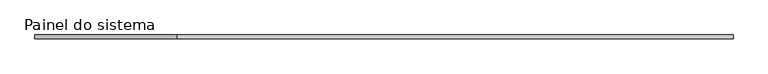
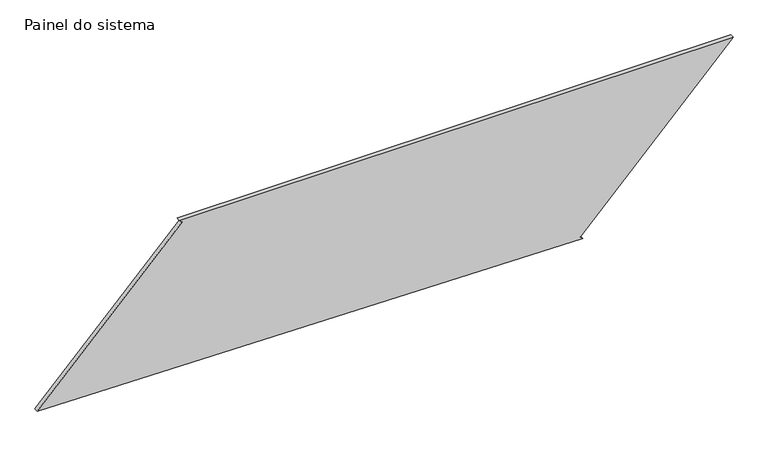
"""IFC4 building model written with IfcOpenShell, lengths in millimetres: plate geometry, Painel do sistema : Envidraçado."""

from ifc_helpers import new_model, si_unit, frame, origin, place, context, project, spatial, polyline, outline, extrude, source, transform, mapped, element, save


def painel_do_sistema_90df6eb1(model_context):
    return source(origin(), model_context, "Body", "SweptSolid", [
        extrude(outline(polyline([(0.0, 1267.032152), (17.3932625, 1249.0745793), (1028.5808351, 2228.4859512), (1028.5808351, -1318.247477), (1011.1875725, -1300.2899043), (52.8769643, -2228.4859512), (0.0, 1267.032152)])), frame((0.0, 24.5, 0.0), z_axis=(0.0, 1.0, 0.0), x_axis=(0.0, 0.0, 1.0)), (0.0, 0.0, 1.0), 25.0),
    ])


if __name__ == "__main__":
    model = new_model("IFC4")
    model_context = context("Model", 3, world=origin())
    ifc_project = project(units=[si_unit("LENGTHUNIT", "METRE", prefix="MILLI")], contexts=[model_context])
    site = spatial("IfcSite", under=ifc_project)
    building = spatial("IfcBuilding", under=site)
    placement = place(None, origin())
    painel_do_sistema_shape = painel_do_sistema_90df6eb1(model_context)
    element("IfcPlate", 1, ObjectType="Painel do sistema : Envidraçado", at=placement, inside=building, context=model_context, shape_type="MappedRepresentation", body=[
        mapped(painel_do_sistema_shape, transform((0.0, 0.0, 0.0), x_axis=(1.0, 0.0, 0.0), y_axis=(0.0, 1.0, 0.0), z_axis=(0.0, 0.0, 1.0))),
    ])
    save(model, "model.ifc")

# Revit data of these elements
# Type "Painel do sistema : Envidraçado"
#   Construction Type Id = "GSP4R"
#   Analytic Construction = "Vidraça única Pilkington 1/8 pol"
#   Visual Light Transmittance = 0.9
#   Solar Heat Gain Coefficient = 0.86
#   Heat Transfer Coefficient (U) = 6.7069 W/(m²·K)
# Element 1 (IfcPlate, "Painel do sistema : Envidraçado")
#   Materials on its faces: "Vidro"
# Materials
#   "Vidro": class "Vidro", colour RGB 0 128 192, transparency 0.9, Description = "Vidro de sílica", Cost = 0
